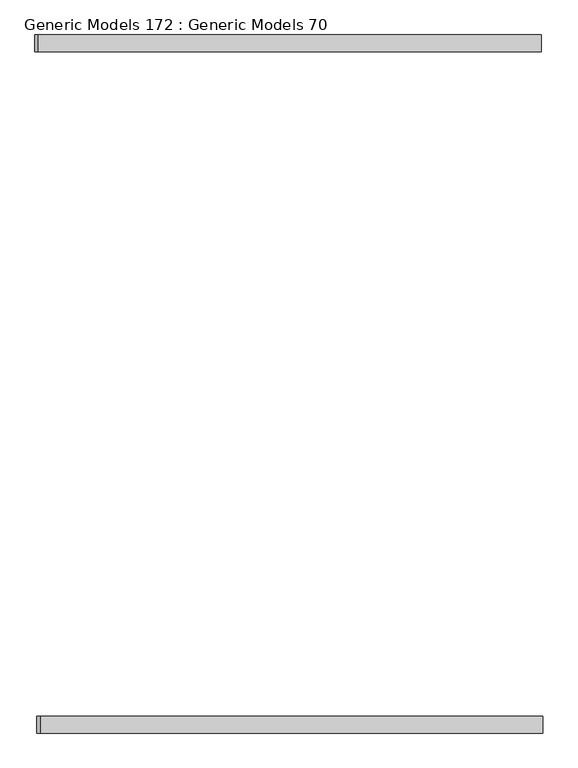
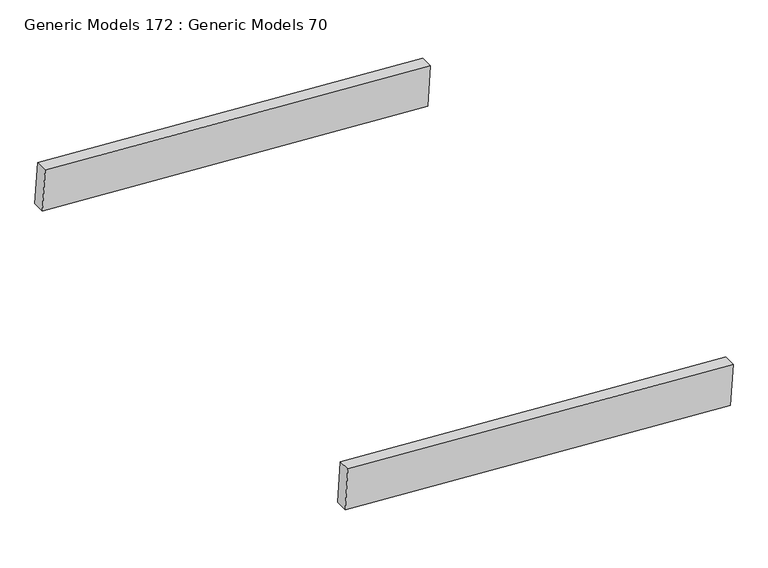
"""IFC4 building model written with IfcOpenShell, lengths in millimetres: proxy geometry, Generic Models 172 : Generic Models 70."""

from ifc_helpers import new_model, si_unit, frame, origin, place, context, project, spatial, polyline, outline, extrude, source, transform, mapped, element, save


def generic_models_172_generic_models_70_ead40be0(model_context):
    return source(origin(), model_context, "Body", "SweptSolid", [
        extrude(outline(polyline([(0.0, -4165.0140379), (0.0, 0.0), (139.7, 0.0), (139.7, -4165.0140379), (0.0, -4165.0140379)])), frame((29915.3947278, 36337.5707942, 271930.8774594), z_axis=(0.062378286155191545, 0.0, 0.9980525784828879), x_axis=(0.0, 1.0, 0.0)), (0.0, 0.0, 1.0), 457.2),
        extrude(outline(polyline([(0.0, -4165.0140379), (0.0, 0.0), (139.7, 0.0), (139.7, -4165.0140379), (0.0, -4165.0140379)])), frame((29929.8137808, 30704.4906612, 271929.9762686), z_axis=(0.06237828615519167, 0.0, 0.9980525784828879), x_axis=(0.0, 1.0, 0.0)), (0.0, 0.0, 1.0), 457.2),
    ])


if __name__ == "__main__":
    model = new_model("IFC4")
    model_context = context("Model", 3, world=origin())
    ifc_project = project(units=[si_unit("LENGTHUNIT", "METRE", prefix="MILLI")], contexts=[model_context])
    site = spatial("IfcSite", under=ifc_project)
    building = spatial("IfcBuilding", under=site)
    placement = place(None, origin())
    generic_models_172_generic_models_70_shape = generic_models_172_generic_models_70_ead40be0(model_context)
    element("IfcBuildingElementProxy", 1, Name="Generic Models 172 : Generic Models 70", ObjectType="Generic Models 172 : Generic Models 70", at=placement, inside=building, context=model_context, shape_type="MappedRepresentation", body=[
        mapped(generic_models_172_generic_models_70_shape, transform((0.0, 0.0, 0.0), x_axis=(1.0, 0.0, 0.0), y_axis=(0.0, 1.0, 0.0), z_axis=(0.0, 0.0, 1.0))),
    ])
    save(model, "model.ifc")

# Revit data of these elements
# Element 1 (IfcBuildingElementProxy, "Generic Models 172 : Generic Models 70")
#   Materials on its faces: "5 1/2\" x 18\" GLULAM BEAM"
# Materials
#   "5 1/2\" x 18\" GLULAM BEAM": class "Wood", colour RGB 112 64 44, transparency 0, Description = "Pinus Echinata", Cost = 0
